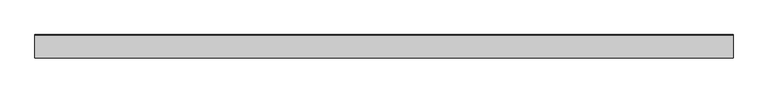
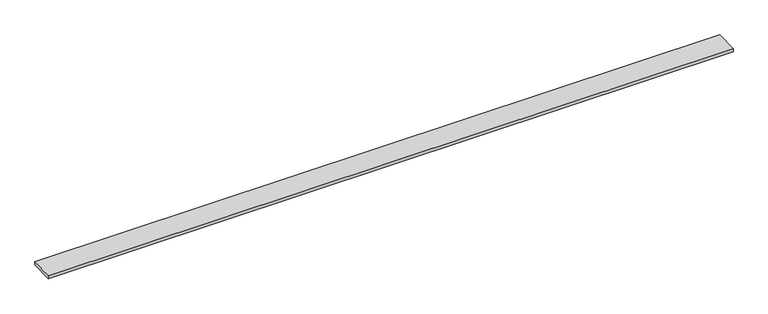
"""IFC4 building model written with IfcOpenShell, lengths in millimetres: proxy geometry, Inner panel:Inner panel:1:Inner panel:1 : Inner panel:Inner panel:300324:2:Inner panel:1:Inner panel:1 : Inner panel:Inner panel:300324:2 : Inner panel:Inner panel:1:Inner panel:1 : Inner panel:Inner panel:300324:300043:9 : Inner panel:Inner panel:1:Inner panel:1 : Inner panel:Inner panel:300324:2:Inner panel:1:Inner panel:1 : Inner panel:Inner panel:300324:2 : Inner panel:Inner panel:1:Inner panel:1 : Inner panel:Inner panel:300324:300043:308120."""

from ifc_helpers import new_model, si_unit, frame, origin, place, context, project, spatial, polyline, outline, extrude, source, transform, mapped, element, save


def generic_models_f4d639fd(model_context):
    return source(origin(), model_context, "Body", "SweptSolid", [
        extrude(outline(polyline([(0.0, -162.2920786), (0.0, 0.0), (4876.8, 0.0), (4876.8, -162.2920786), (0.0, -162.2920786)])), frame((596182.8367242, -536656.4713008, 10095.7995008), z_axis=(0.0, -0.04163054471218133, 0.999133073092352), x_axis=(-1.0, 0.0, 0.0)), (0.0, 0.0, 1.0), 21.6347684),
    ])


if __name__ == "__main__":
    model = new_model("IFC4")
    model_context = context("Model", 3, world=origin())
    ifc_project = project(units=[si_unit("LENGTHUNIT", "METRE", prefix="MILLI")], contexts=[model_context])
    site = spatial("IfcSite", under=ifc_project)
    building = spatial("IfcBuilding", under=site)
    placement = place(None, origin())
    generic_models_shape = generic_models_f4d639fd(model_context)
    element("IfcBuildingElementProxy", 1, Name="Inner panel:Inner panel:1:Inner panel:1 : Inner panel:Inner panel:300324:2:Inner panel:1:Inner panel:1 : Inner panel:Inner panel:300324:2 : Inner panel:Inner panel:1:Inner panel:1 : Inner panel:Inner panel:300324:300043:9 : Inner panel:Inner panel:1:Inner panel:1 : Inner panel:Inner panel:300324:2:Inner panel:1:Inner panel:1 : Inner panel:Inner panel:300324:2 : Inner panel:Inner panel:1:Inner panel:1 : Inner panel:Inner panel:300324:300043:308120", ObjectType="Inner panel:Inner panel:1:Inner panel:1 : Inner panel:Inner panel:300324:2:Inner panel:1:Inner panel:1 : Inner panel:Inner panel:300324:2 : Inner panel:Inner panel:1:Inner panel:1 : Inner panel:Inner panel:300324:300043:9 : Inner panel:Inner panel:1:Inner panel:1 : Inner panel:Inner panel:300324:2:Inner panel:1:Inner panel:1 : Inner panel:Inner panel:300324:2 : Inner panel:Inner panel:1:Inner panel:1 : Inner panel:Inner panel:300324:300043:308120", at=placement, inside=building, context=model_context, shape_type="MappedRepresentation", body=[
        mapped(generic_models_shape, transform((0.0, 0.0, 0.0), x_axis=(1.0, 0.0, 0.0), y_axis=(0.0, 1.0, 0.0), z_axis=(0.0, 0.0, 1.0))),
    ])
    save(model, "model.ifc")

# Revit data of these elements
# Type "Inner panel:Inner panel:1:Inner panel:1 : Inner panel:Inner panel:300324:2:Inner panel:1:Inner panel:1 : Inner panel:Inner panel:300324:2 : Inner panel:Inner panel:1:Inner panel:1 : Inner panel:Inner panel:300324:300043:9 : Inner panel:Inner panel:1:Inner panel:1 : Inner panel:Inner panel:300324:2:Inner panel:1:Inner panel:1 : Inner panel:Inner panel:300324:2 : Inner panel:Inner panel:1:Inner panel:1 : Inner panel:Inner panel:300324:300043:308120"
#   NameOverride = "Inner panel:Inner panel:1:Inner panel:1 : Inner panel:Inner panel:300324:2:Inner panel:1:Inner panel:1 : Inner panel:Inner panel:300324:2 : Inner panel:Inner panel:1:Inner panel:1 : Inner panel:Inner panel:300324:300043:308120"
#   ObjectTypeOverride = "Inner panel:1:Inner panel:1 : Inner panel:Inner panel:300324:2 : Inner panel:Inner panel:1:Inner panel:1 : Inner panel:Inner panel:300324:300043"
#   Reference = "Inner panel"
#   Tag = "308120"
# Element 1 (IfcBuildingElementProxy, "Inner panel:Inner panel:1:Inner panel:1 : Inner panel:Inner panel:300324:2:Inner panel:1:Inner panel:1 : Inner panel:Inner panel:300324:2 : Inner panel:Inner panel:1:Inner panel:1 : Inner panel:Inner panel:300324:300043:9 : Inner panel:Inner panel:1:Inner panel:1 : Inner panel:Inner panel:300324:2:Inner panel:1:Inner panel:1 : Inner panel:Inner panel:300324:2 : Inner panel:Inner panel:1:Inner panel:1 : Inner panel:Inner panel:300324:300043:308120")
#   Materials on its faces: "1\" THERMAL SPACER @ PURLIN"
# Materials
#   "1\" THERMAL SPACER @ PURLIN": class "Unassigned", colour RGB 205 188 106, transparency 0, Cost = 0
